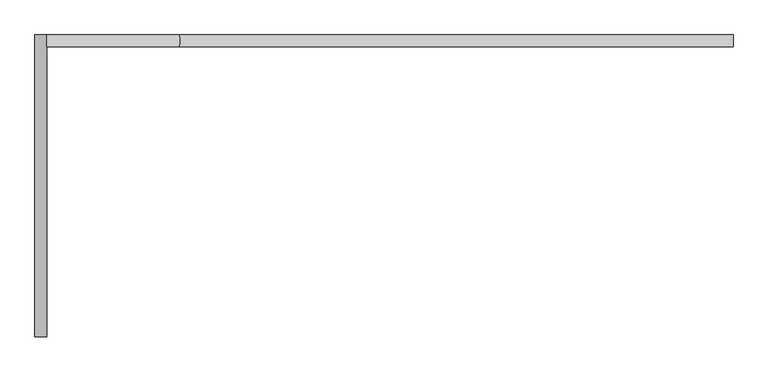
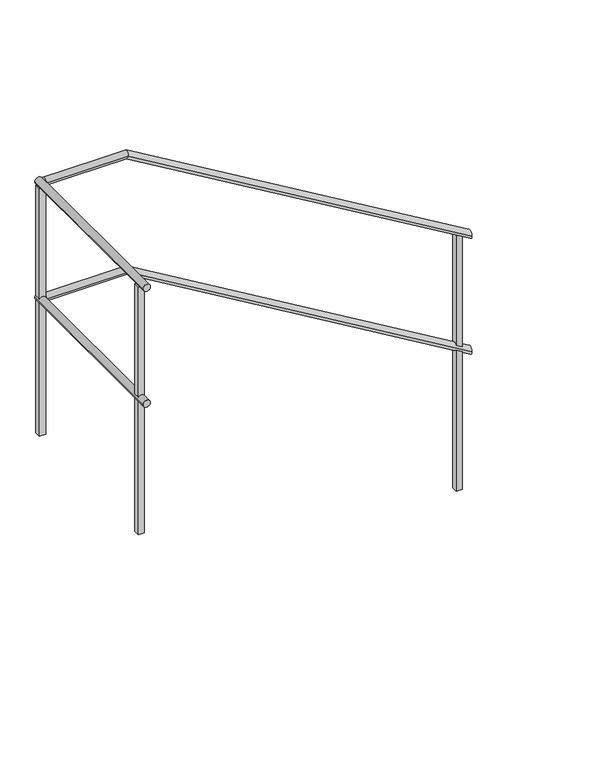
"""IFC4 building model written with IfcOpenShell, lengths in millimetres: railing geometry."""

from ifc_helpers import new_model, si_unit, frame, origin, place, context, project, spatial, polyline, circle_curve, ellipse_curve, outline, extrude, source, transform, mapped, element, save
from ifc_brep_helpers import plane_surface, cylinder_surface, advanced_brep


def railing_f9e899a6(model_context):
    return source(origin(), model_context, "Body", "SolidModel", [
        advanced_brep(
        [(33043.8956602, 24484.5208589, 899.1723166), (33043.8956602, 24514.5208589, 899.1723166), (31639.7692216, 24484.5208589, 1734.9618634), (31639.7692216, 24514.5208589, 1734.9618634), (31305.4, 24484.5208589, 1734.9618634), (31305.4, 24514.5208589, 1734.9618634)],
        [
            (0, 1, ellipse_curve(frame((33043.8956602, 24499.5208589, 899.1723166), z_axis=(1.0, 0.0, 0.0), x_axis=(0.0, 0.0, -1.0)), 17.4562134, 15.0)),
            (1, 0, ellipse_curve(frame((33043.8956602, 24499.5208589, 899.1723166), z_axis=(1.0, 0.0, 0.0), x_axis=(0.0, 0.0, -1.0)), 17.4562134, 15.0)),
            (0, 2),
            (2, 3, ellipse_curve(frame((31639.7692216, 24499.5208589, 1734.9618634), z_axis=(0.9641817474962141, 0.0, -0.2652424509673118), x_axis=(-0.26524245096731197, 0.0, -0.9641817474962142)), 15.5572329, 15.0)),
            (3, 1),
            (3, 2, ellipse_curve(frame((31639.7692216, 24499.5208589, 1734.9618634), z_axis=(0.9641817474962141, 0.0, -0.2652424509673118), x_axis=(-0.26524245096731197, 0.0, -0.9641817474962142)), 15.5572329, 15.0)),
            (4, 5, circle_curve(frame((31305.4, 24499.5208589, 1734.9618634), z_axis=(-1.0, 0.0, 0.0), x_axis=(0.0, 1.0, 0.0)), 15.0)),
            (5, 4, circle_curve(frame((31305.4, 24499.5208589, 1734.9618634), z_axis=(-1.0, 0.0, 0.0), x_axis=(0.0, 1.0, 0.0)), 15.0)),
            (2, 4),
            (5, 3),
        ],
        [
            plane_surface(frame((33043.8956602, 24499.5208589, 916.62853), z_axis=(1.0, 0.0, 0.0), x_axis=(0.0, -1.0, 0.0))),
            cylinder_surface(frame((33036.2234023, 24499.5208589, 903.7391368), z_axis=(0.8592928844097064, 0.0, -0.5114838597676832), x_axis=(0.0, 1.0, 0.0)), 15.0),
            plane_surface(frame((31305.4, 24499.5208589, 1749.9618634), z_axis=(-1.0, 0.0, 0.0), x_axis=(0.0, -1.0, 0.0))),
            cylinder_surface(frame((31643.8956602, 24499.5208589, 1734.9618634), z_axis=(1.0, 0.0, 0.0), x_axis=(0.0, 1.0, 0.0)), 15.0),
        ],
        [
            (0, [[1, 2]]),
            (1, [[-1, 3, 4, 5]]),
            (1, [[-2, -5, 6, -3]]),
            (2, [[7, 8]]),
            (3, [[-4, 9, -8, 10]]),
            (3, [[-6, -10, -7, -9]]),
        ],
    ),
        advanced_brep(
        [(33043.8956602, 24484.5208589, 1399.1723166), (33043.8956602, 24514.5208589, 1399.1723166), (31639.7692216, 24484.5208589, 2234.9618634), (31639.7692216, 24514.5208589, 2234.9618634), (31305.4, 24484.5208589, 2234.9618634), (31305.4, 24514.5208589, 2234.9618634)],
        [
            (0, 1, ellipse_curve(frame((33043.8956602, 24499.5208589, 1399.1723166), z_axis=(1.0, 0.0, 0.0), x_axis=(0.0, 0.0, -1.0)), 17.4562134, 15.0)),
            (1, 0, ellipse_curve(frame((33043.8956602, 24499.5208589, 1399.1723166), z_axis=(1.0, 0.0, 0.0), x_axis=(0.0, 0.0, -1.0)), 17.4562134, 15.0)),
            (0, 2),
            (2, 3, ellipse_curve(frame((31639.7692216, 24499.5208589, 2234.9618634), z_axis=(0.9641817474962141, 0.0, -0.2652424509673118), x_axis=(-0.26524245096731197, 0.0, -0.9641817474962142)), 15.5572329, 15.0)),
            (3, 1),
            (3, 2, ellipse_curve(frame((31639.7692216, 24499.5208589, 2234.9618634), z_axis=(0.9641817474962141, 0.0, -0.2652424509673118), x_axis=(-0.26524245096731197, 0.0, -0.9641817474962142)), 15.5572329, 15.0)),
            (4, 5, circle_curve(frame((31305.4, 24499.5208589, 2234.9618634), z_axis=(-1.0, 0.0, 0.0), x_axis=(0.0, 1.0, 0.0)), 15.0)),
            (5, 4, circle_curve(frame((31305.4, 24499.5208589, 2234.9618634), z_axis=(-1.0, 0.0, 0.0), x_axis=(0.0, 1.0, 0.0)), 15.0)),
            (2, 4),
            (5, 3),
        ],
        [
            plane_surface(frame((33043.8956602, 24499.5208589, 1416.62853), z_axis=(1.0, 0.0, 0.0), x_axis=(0.0, -1.0, 0.0))),
            cylinder_surface(frame((33036.2234023, 24499.5208589, 1403.7391368), z_axis=(0.8592928844097064, 0.0, -0.5114838597676832), x_axis=(0.0, 1.0, 0.0)), 15.0),
            plane_surface(frame((31305.4, 24499.5208589, 2249.9618634), z_axis=(-1.0, 0.0, 0.0), x_axis=(0.0, -1.0, 0.0))),
            cylinder_surface(frame((31643.8956602, 24499.5208589, 2234.9618634), z_axis=(1.0, 0.0, 0.0), x_axis=(0.0, 1.0, 0.0)), 15.0),
        ],
        [
            (0, [[1, 2]]),
            (1, [[-1, 3, 4, 5]]),
            (1, [[-2, -5, 6, -3]]),
            (2, [[7, 8]]),
            (3, [[-4, 9, -8, 10]]),
            (3, [[-6, -10, -7, -9]]),
        ],
    ),
        advanced_brep(
        [(31305.4, 24514.5208589, 1734.9618634), (31275.4, 24514.5208589, 1734.9618634), (31305.4, 23749.5208589, 1734.9618634), (31275.4, 23749.5208589, 1734.9618634)],
        [
            (0, 1, circle_curve(frame((31290.4, 24514.5208589, 1734.9618634), z_axis=(0.0, 1.0, 0.0), x_axis=(-1.0, 0.0, 0.0)), 15.0)),
            (1, 0, circle_curve(frame((31290.4, 24514.5208589, 1734.9618634), z_axis=(0.0, 1.0, 0.0), x_axis=(-1.0, 0.0, 0.0)), 15.0)),
            (2, 3, circle_curve(frame((31290.4, 23749.5208589, 1734.9618634), z_axis=(0.0, -1.0, 0.0), x_axis=(-1.0, 0.0, 0.0)), 15.0)),
            (3, 2, circle_curve(frame((31290.4, 23749.5208589, 1734.9618634), z_axis=(0.0, -1.0, 0.0), x_axis=(-1.0, 0.0, 0.0)), 15.0)),
            (0, 2),
            (3, 1),
        ],
        [
            plane_surface(frame((31290.4, 24514.5208589, 1749.9618634), z_axis=(0.0, 1.0, 0.0), x_axis=(0.0, 0.0, -1.0))),
            plane_surface(frame((31290.4, 23749.5208589, 1749.9618634), z_axis=(0.0, -1.0, 0.0), x_axis=(0.0, 0.0, -1.0))),
            cylinder_surface(frame((31290.4, 24514.5208589, 1734.9618634), z_axis=(0.0, 1.0, 0.0), x_axis=(-1.0, 0.0, 0.0)), 15.0),
        ],
        [
            (0, [[1, 2]]),
            (1, [[3, 4]]),
            (2, [[-1, 5, -4, 6]]),
            (2, [[-2, -6, -3, -5]]),
        ],
    ),
        advanced_brep(
        [(31305.4, 24514.5208589, 2234.9618634), (31275.4, 24514.5208589, 2234.9618634), (31305.4, 23749.5208589, 2234.9618634), (31275.4, 23749.5208589, 2234.9618634)],
        [
            (0, 1, circle_curve(frame((31290.4, 24514.5208589, 2234.9618634), z_axis=(0.0, 1.0, 0.0), x_axis=(-1.0, 0.0, 0.0)), 15.0)),
            (1, 0, circle_curve(frame((31290.4, 24514.5208589, 2234.9618634), z_axis=(0.0, 1.0, 0.0), x_axis=(-1.0, 0.0, 0.0)), 15.0)),
            (2, 3, circle_curve(frame((31290.4, 23749.5208589, 2234.9618634), z_axis=(0.0, -1.0, 0.0), x_axis=(-1.0, 0.0, 0.0)), 15.0)),
            (3, 2, circle_curve(frame((31290.4, 23749.5208589, 2234.9618634), z_axis=(0.0, -1.0, 0.0), x_axis=(-1.0, 0.0, 0.0)), 15.0)),
            (0, 2),
            (3, 1),
        ],
        [
            plane_surface(frame((31290.4, 24514.5208589, 2249.9618634), z_axis=(0.0, 1.0, 0.0), x_axis=(0.0, 0.0, -1.0))),
            plane_surface(frame((31290.4, 23749.5208589, 2249.9618634), z_axis=(0.0, -1.0, 0.0), x_axis=(0.0, 0.0, -1.0))),
            cylinder_surface(frame((31290.4, 24514.5208589, 2234.9618634), z_axis=(0.0, 1.0, 0.0), x_axis=(-1.0, 0.0, 0.0)), 15.0),
        ],
        [
            (0, [[1, 2]]),
            (1, [[3, 4]]),
            (2, [[-1, 5, -4, 6]]),
            (2, [[-2, -6, -3, -5]]),
        ],
    ),
        extrude(outline(polyline([(31302.9, 24512.0208589), (31302.9, 24487.0208589), (31277.9, 24487.0208589), (31277.9, 24512.0208589), (31302.9, 24512.0208589)])), frame((0.0, 0.0, 1149.9618634), z_axis=(0.0, 0.0, 1.0), x_axis=(1.0, 0.0, 0.0)), (0.0, 0.0, 1.0), 1070.0),
        extrude(outline(polyline([(31277.9, 23812.0208589), (31302.9, 23812.0208589), (31302.9, 23787.0208589), (31277.9, 23787.0208589), (31277.9, 23812.0208589)])), frame((0.0, 0.0, 1149.9618634), z_axis=(0.0, 0.0, 1.0), x_axis=(1.0, 0.0, 0.0)), (0.0, 0.0, 1.0), 1070.0),
        extrude(outline(polyline([(316.62853, 33006.3956602), (1408.9499586, 33006.3956602), (1423.830911, 32981.3956602), (316.62853, 32981.3956602), (316.62853, 33006.3956602)])), frame((0.0, 24487.0208589, 0.0), z_axis=(0.0, 1.0, 0.0), x_axis=(0.0, 0.0, 1.0)), (0.0, 0.0, 1.0), 25.0),
    ])


if __name__ == "__main__":
    model = new_model("IFC4")
    model_context = context("Model", 3, world=origin())
    ifc_project = project(units=[si_unit("LENGTHUNIT", "METRE", prefix="MILLI")], contexts=[model_context])
    site = spatial("IfcSite", under=ifc_project)
    building = spatial("IfcBuilding", under=site)
    placement = place(None, origin())
    railing_shape = railing_f9e899a6(model_context)
    element("IfcRailing", 1, at=placement, inside=building, context=model_context, shape_type="MappedRepresentation", body=[
        mapped(railing_shape, transform((0.0, 0.0, 0.0), x_axis=(1.0, 0.0, 0.0), y_axis=(0.0, 1.0, 0.0), z_axis=(0.0, 0.0, 1.0))),
    ])
    save(model, "model.ifc")
